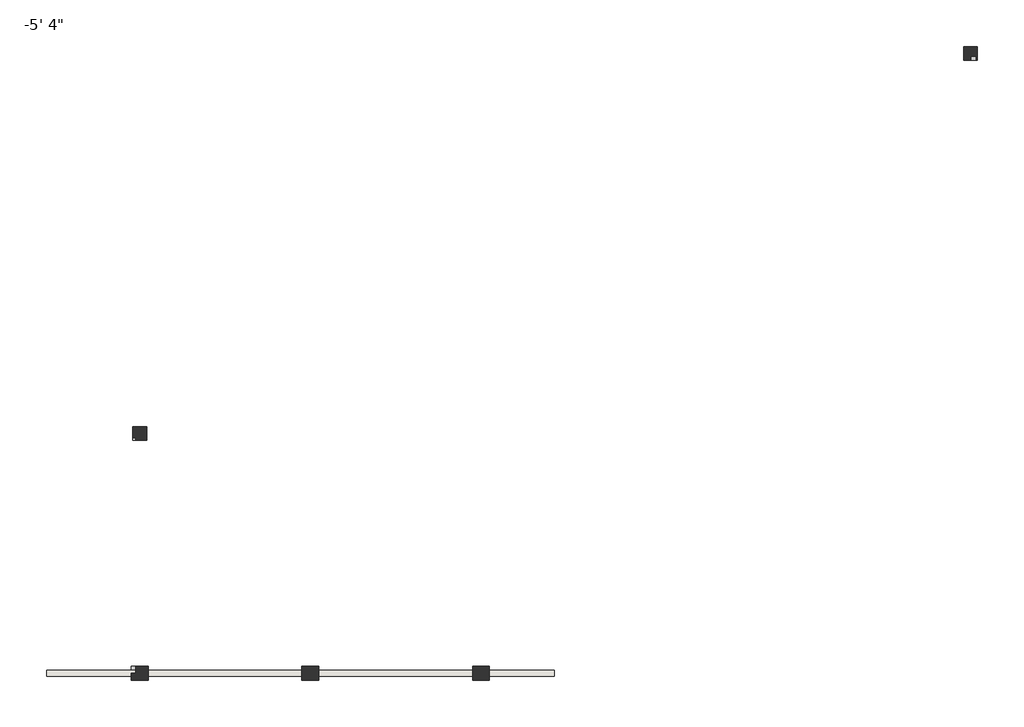
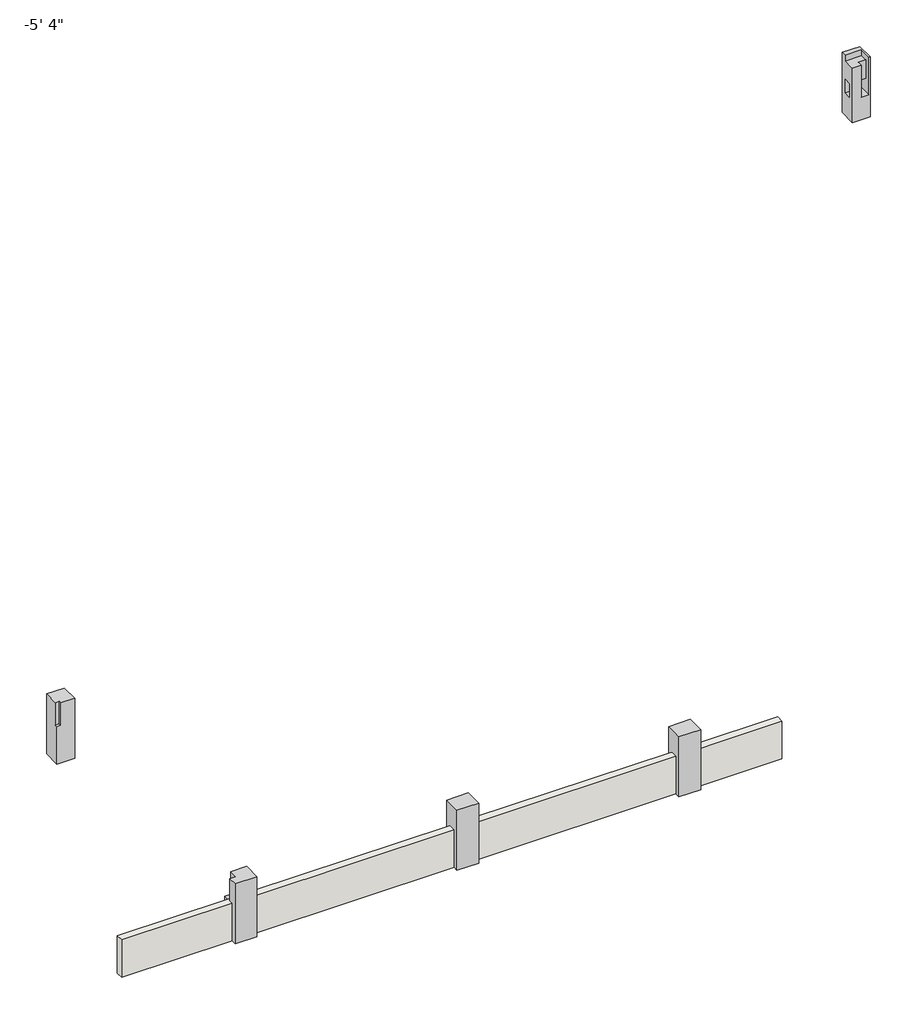
# One storey: 5 columns, 1 wall.
"""IFC4 building model written with IfcOpenShell, lengths in millimetres."""

from ifc_helpers import new_model, si_unit, frame, origin, place, context, project, spatial, polyline, outline, extrude, faceted_brep, element, save

model = new_model("IFC4")

# Units and contexts
model_context = context("Model", 3, world=origin())
ifc_project = project(units=[si_unit("LENGTHUNIT", "METRE", prefix="MILLI")], contexts=[model_context])

# Site, building, storey
site = spatial("IfcSite", under=ifc_project)
building = spatial("IfcBuilding", under=site)
storey = spatial("IfcBuildingStorey", under=building, Name="-5' 4\"", Elevation=-1625.6)

# Columns
placement = place(None, origin())
element("IfcColumn", 1, ObjectType="Concrete-Rectangular-Column : P1", at=placement, inside=storey, context=model_context, shape_type="Brep", body=[
    faceted_brep([(718.2325311, 9347.3676661, -1625.6), (718.2325311, 8890.1676661, -1625.6), (261.0325311, 8890.1676661, -1625.6), (261.0325311, 9347.3676661, -1625.6), (718.2325311, 9347.3676661, 0.0), (718.2325311, 8890.1676661, 0.0), (683.3075311, 8890.1676661, 0.0), (683.3075311, 8890.1676661, -1016.0), (489.6325311, 8890.1676661, -1016.0), (489.6325311, 8890.1676661, -152.4), (261.0325311, 8890.1676661, -152.4), (261.0325311, 9215.6051661, -152.4), (261.0325311, 9215.6051661, 0.0), (261.0325311, 9347.3676661, 0.0), (261.0325311, 9021.9301661, -647.7), (261.0325311, 9021.9301661, -1016.0), (261.0325311, 9215.6051661, -1016.0), (261.0325311, 9215.6051661, -647.7), (683.3075311, 9215.6051661, 0.0), (683.3075311, 9021.9301661, 0.0), (683.3075311, 9215.6051661, -152.4), (489.6325311, 9021.9301661, -152.4), (683.3075311, 9021.9301661, -152.4), (683.3075311, 9021.9301661, -647.7), (683.3075311, 9215.6051661, -647.7), (683.3075311, 9215.6051661, -1016.0), (683.3075311, 9021.9301661, -1016.0), (489.6325311, 9021.9301661, -647.7), (489.6325311, 9021.9301661, -1016.0)], [[[0, 1, 2, 3]], [[1, 0, 4, 5]], [[2, 1, 5, 6, 7, 8, 9, 10]], [[3, 2, 10, 11, 12, 13], [14, 15, 16, 17]], [[0, 3, 13, 4]], [[5, 4, 13, 12, 18, 19, 6]], [[20, 11, 10, 9, 21, 22]], [[18, 20, 22, 23, 24, 25, 26, 7, 6, 19]], [[20, 18, 12, 11]], [[15, 14, 27, 28]], [[25, 24, 17, 16]], [[7, 26, 25, 16, 15, 28, 8]], [[24, 23, 27, 14, 17]], [[27, 21, 9, 8, 28]], [[23, 22, 21, 27]]]),
])
element("IfcColumn", 2, ObjectType="Concrete-Rectangular-Column : P1", at=placement, inside=storey, context=model_context, shape_type="Brep", body=[
    faceted_brep([(-26993.1674689, -3327.2323339, -1625.6), (-26993.1674689, -3784.4323339, -1625.6), (-27450.3674689, -3784.4323339, -1625.6), (-27450.3674689, -3327.2323339, -1625.6), (-26993.1674689, -3327.2323339, 0.0), (-26993.1674689, -3784.4323339, 0.0), (-27348.7674689, -3784.4323339, 0.0), (-27348.7674689, -3784.4323339, -609.6), (-27450.3674689, -3784.4323339, -609.6), (-27450.3674689, -3708.2323339, -609.6), (-27450.3674689, -3708.2323339, 0.0), (-27450.3674689, -3327.2323339, 0.0), (-27348.7674689, -3708.2323339, 0.0), (-27348.7674689, -3708.2323339, -609.6)], [[[0, 1, 2, 3]], [[1, 0, 4, 5]], [[2, 1, 5, 6, 7, 8]], [[3, 2, 8, 9, 10, 11]], [[0, 3, 11, 4]], [[5, 4, 11, 10, 12, 6]], [[9, 13, 12, 10]], [[13, 9, 8, 7]], [[12, 13, 7, 6]]]),
])
element("IfcColumn", 3, ObjectType="Concrete-Rectangular-Column : P2", at=placement, inside=storey, context=model_context, shape_type="SweptSolid", body=[
    extrude(outline(polyline([(-11785.4323339, -1625.6), (-11785.4323339, 0.0), (-11328.2323339, 0.0), (-11328.2323339, -1625.6), (-11459.9948339, -1625.6), (-11459.9948339, -609.6), (-11653.6698339, -609.6), (-11653.6698339, -1625.6), (-11785.4323339, -1625.6)])), frame((-16121.9674689, 0.0, 0.0), z_axis=(1.0, 0.0, 0.0), x_axis=(0.0, 1.0, 0.0)), (0.0, 0.0, 1.0), 558.8),
])
element("IfcColumn", 4, ObjectType="Concrete-Rectangular-Column : P2", at=placement, inside=storey, context=model_context, shape_type="SweptSolid", body=[
    extrude(outline(polyline([(-11785.4323339, -1625.6), (-11785.4323339, 0.0), (-11328.2323339, 0.0), (-11328.2323339, -1625.6), (-11459.9948339, -1625.6), (-11459.9948339, -609.6), (-11653.6698339, -609.6), (-11653.6698339, -1625.6), (-11785.4323339, -1625.6)])), frame((-21811.5674689, 0.0, 0.0), z_axis=(1.0, 0.0, 0.0), x_axis=(0.0, 1.0, 0.0)), (0.0, 0.0, 1.0), 558.8),
])
element("IfcColumn", 5, ObjectType="Concrete-Rectangular-Column : P2", at=placement, inside=storey, context=model_context, shape_type="Brep", body=[
    faceted_brep([(-27501.1674689, -11328.2323339, -1625.6), (-26942.3674689, -11328.2323339, -1625.6), (-26942.3674689, -11459.9948339, -1625.6), (-27501.1674689, -11459.9948339, -1625.6), (-26942.3674689, -11328.2323339, 0.0), (-26942.3674689, -11785.4323339, 0.0), (-26942.3674689, -11785.4323339, -1625.6), (-26942.3674689, -11653.6698339, -1625.6), (-26942.3674689, -11653.6698339, -609.6), (-26942.3674689, -11459.9948339, -609.6), (-27501.1674689, -11785.4323339, -1625.6), (-27501.1674689, -11785.4323339, 0.0), (-27501.1674689, -11556.8323339, 0.0), (-27501.1674689, -11556.8323339, -609.6), (-27501.1674689, -11653.6698339, -609.6), (-27501.1674689, -11653.6698339, -1625.6), (-27501.1674689, -11328.2323339, -609.6), (-27348.7674689, -11328.2323339, -609.6), (-27348.7674689, -11328.2323339, 0.0), (-27348.7674689, -11556.8323339, 0.0), (-27348.7674689, -11459.9948339, -609.6), (-27501.1674689, -11459.9948339, -609.6), (-27348.7674689, -11556.8323339, -609.6)], [[[0, 1, 2, 3]], [[4, 5, 6, 7, 8, 9, 2, 1]], [[10, 6, 5, 11]], [[10, 11, 12, 13, 14, 15]], [[1, 0, 16, 17, 18, 4]], [[5, 4, 18, 19, 12, 11]], [[3, 2, 9, 20, 21]], [[14, 8, 7, 15]], [[8, 14, 13, 22, 20, 9]], [[6, 10, 15, 7]], [[17, 20, 22, 19, 18]], [[20, 17, 16, 21]], [[19, 22, 13, 12]], [[0, 3, 21, 16]]]),
])

# Wall
element("IfcWall", 6, ObjectType="Generic - 8\" Masonry", at=placement, inside=storey, context=model_context, shape_type="Brep", body=[
    faceted_brep([(-13404.1674689, -11459.9948339, -1625.6), (-15563.1674689, -11459.9948339, -1625.6), (-16121.9674689, -11459.9948339, -1625.6), (-21252.7674689, -11459.9948339, -1625.6), (-21811.5674689, -11459.9948339, -1625.6), (-26942.3674689, -11459.9948339, -1625.6), (-27501.1674689, -11459.9948339, -1625.6), (-30330.0924689, -11459.9948339, -1625.6), (-30330.0924689, -11459.9948339, -609.6), (-27501.1674689, -11459.9948339, -609.6), (-27348.7674689, -11459.9948339, -609.6), (-26942.3674689, -11459.9948339, -609.6), (-21811.5674689, -11459.9948339, -609.6), (-21252.7674689, -11459.9948339, -609.6), (-16121.9674689, -11459.9948339, -609.6), (-15563.1674689, -11459.9948339, -609.6), (-13404.1674689, -11459.9948339, -609.6), (-13404.1674689, -11653.6698339, -1625.6), (-13404.1674689, -11653.6698339, -609.6), (-15563.1674689, -11653.6698339, -609.6), (-16121.9674689, -11653.6698339, -609.6), (-21252.7674689, -11653.6698339, -609.6), (-21811.5674689, -11653.6698339, -609.6), (-26942.3674689, -11653.6698339, -609.6), (-27501.1674689, -11653.6698339, -609.6), (-30330.0924689, -11653.6698339, -609.6), (-30330.0924689, -11653.6698339, -1625.6), (-27501.1674689, -11653.6698339, -1625.6), (-26942.3674689, -11653.6698339, -1625.6), (-21811.5674689, -11653.6698339, -1625.6), (-21252.7674689, -11653.6698339, -1625.6), (-16121.9674689, -11653.6698339, -1625.6), (-15563.1674689, -11653.6698339, -1625.6)], [[[0, 1, 2, 3, 4, 5, 6, 7, 8, 9, 10, 11, 12, 13, 14, 15, 16]], [[17, 18, 19, 20, 21, 22, 23, 24, 25, 26, 27, 28, 29, 30, 31, 32]], [[7, 6, 5, 4, 3, 2, 1, 0, 17, 32, 31, 30, 29, 28, 27, 26]], [[16, 15, 14, 13, 12, 11, 10, 9, 8, 25, 24, 23, 22, 21, 20, 19, 18]], [[0, 16, 18, 17]], [[8, 7, 26, 25]]]),
])

save(model, "model.ifc")

# Revit data of these elements
# Type "Concrete-Rectangular-Column : P1"
#   Assembly Code = "B10"
#   b = 1' - 6"
#   h = 1' - 6"
#   Structural Material [instance default] = Concrete, Cast-in-Place gray
# Type "Concrete-Rectangular-Column : P2"
#   Assembly Code = "B10"
#   b = 1' - 10"
#   h = 1' - 6"
#   Structural Material [instance default] = Concrete, Cast-in-Place gray
# Type "Generic - 8\" Masonry"
#   Assembly Code = "B2010"
#   Layers, outside or top first: 0' - 7 5/8" "Concrete Masonry Units" (function 1)
# Elements 1, 2 (IfcColumn, "Concrete-Rectangular-Column : P1")
#   Comments = ""
#   Structural Material = Concrete, Cast-in-Place gray
#   Phase Created = New Construction
#   Materials on its faces: "Concrete, Cast-in-Place gray"
# Elements 3, 4, 5 (IfcColumn, "Concrete-Rectangular-Column : P2")
#   Comments = ""
#   Structural Material = Concrete, Cast-in-Place gray
#   Phase Created = New Construction
#   Materials on its faces: "Concrete, Cast-in-Place gray"
# Element 6 (IfcWall, "Generic - 8\" Masonry")
#   Comments = ""
#   Top Offset = 0' - 0"
#   Base Offset = 0' - 0"
#   wall height = 3' - 4"
#   Phase Created = New Construction
#   Base Constraint = -5' 4"
#   Top Constraint = Lower Floor
#   Materials on its faces: "Concrete Masonry Units"
# Materials
#   "Concrete, Cast-in-Place gray": class "Concrete", colour RGB 192 192 192, transparency 0, Description = "Cast-in-place concrete", Cost = 0
#   "Concrete Masonry Units": class "Masonry", colour RGB 227 227 227, transparency 0, Description = "Concrete masonry units", Cost = 0
